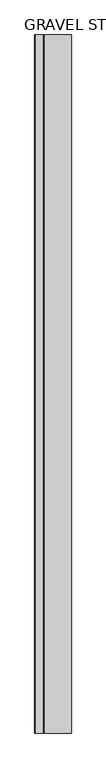
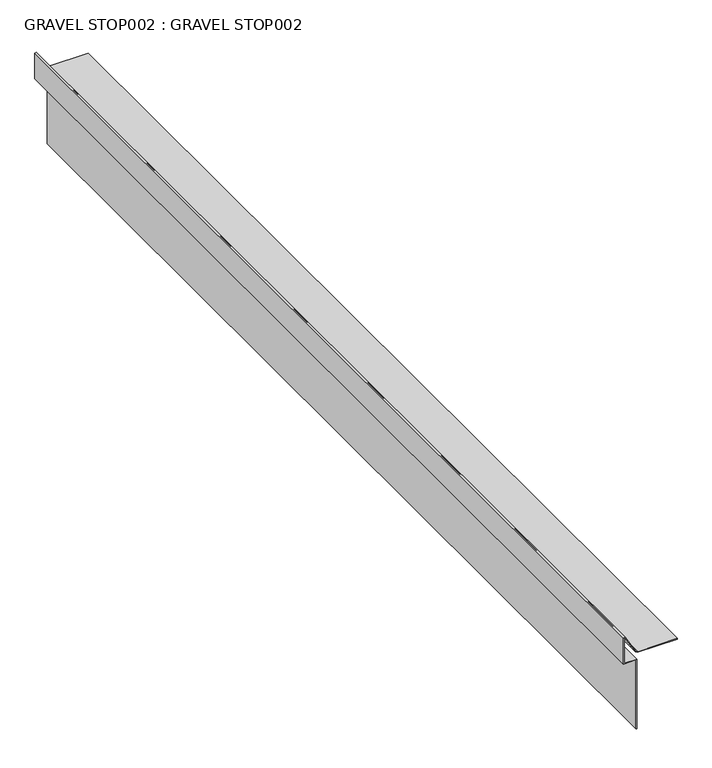
"""IFC4 building model written with IfcOpenShell, lengths in millimetres: proxy geometry, GRAVEL STOP002 : GRAVEL STOP002."""

import ifcopenshell
import ifcopenshell.guid

model = None  # the IFC model being written
_history = None  # IfcOwnerHistory: only IFC2X3 demands one
_inside = {}  # id of a spatial element -> (the spatial element, [elements in it])
_under = {}  # id of a project, library or spatial element -> (it, [spatial elements below it])
_declared = {}  # id of a project -> (the project, [libraries it declares])
_typed = {}  # id of a type object -> (the type object, [elements of that type])
_made_of = {}  # id of a material, layer set ... -> (it, [elements and type objects made of it])


def new_model(schema):
    """Start an empty IFC model of exactly this schema.

    Asked for "IFC4X3", IfcOpenShell would pick the latest addendum, in which some entities
    have other attributes; the version numbers below select the first issue.
    IFC2X3 requires an IfcOwnerHistory on every rooted entity: one is made here for all.
    """
    global model, _history
    if schema == "IFC4X3":
        model = ifcopenshell.file(schema_version=(4, 3, 0, 0))
    else:
        model = ifcopenshell.file(schema=schema)
    _inside.clear()
    _under.clear()
    _declared.clear()
    _typed.clear()
    _made_of.clear()
    _history = None
    if model.schema == "IFC2X3":
        org = make("IfcOrganization", Name="unknown")
        user = make(
            "IfcPersonAndOrganization",
            ThePerson=make("IfcPerson", FamilyName="unknown"),
            TheOrganization=org,
        )
        app = make(
            "IfcApplication",
            ApplicationDeveloper=org,
            Version="unknown",
            ApplicationFullName="unknown",
            ApplicationIdentifier="unknown",
        )
        _history = make(
            "IfcOwnerHistory",
            OwningUser=user,
            OwningApplication=app,
            ChangeAction="ADDED",
            CreationDate=0,
        )
    return model


def make(cls, **values):
    """One entity of the class cls with the attributes given. An attribute that is None is left unset."""
    return model.create_entity(
        cls, **{name: value for name, value in values.items() if value is not None}
    )


def rooted(cls, **values):
    """An entity with a GlobalId (a new one), such as an element, a storey or a relation."""
    return make(cls, GlobalId=ifcopenshell.guid.new(), OwnerHistory=_history, **values)


def si_unit(unit_type, name, prefix=None):
    """IfcSIUnit, for example si_unit("LENGTHUNIT", "METRE", prefix="MILLI")."""
    return make("IfcSIUnit", UnitType=unit_type, Prefix=prefix, Name=name)


def assignment(units):
    """IfcUnitAssignment: the units of a project."""
    return None if units is None else make("IfcUnitAssignment", Units=units)


def point(xyz):
    """IfcCartesianPoint."""
    return None if xyz is None else make("IfcCartesianPoint", Coordinates=xyz)


def direction(xyz):
    """IfcDirection."""
    return None if xyz is None else make("IfcDirection", DirectionRatios=xyz)


def frame(location, z_axis=None, x_axis=None):
    """IfcAxis2Placement3D, a coordinate frame: its origin and axes. An axis left out is left unset."""
    return make(
        "IfcAxis2Placement3D",
        Location=point(location),
        Axis=direction(z_axis),
        RefDirection=direction(x_axis),
    )


def origin():
    """The frame at (0, 0, 0) with its axes left unset."""
    return frame((0.0, 0.0, 0.0))


def place(relative_to, where):
    """IfcLocalPlacement: puts the frame where relative to a parent placement (None: the world)."""
    return make(
        "IfcLocalPlacement", PlacementRelTo=relative_to, RelativePlacement=where
    )


def context(
    kind, dimensions, precision=None, world=None, true_north=None, identifier=None
):
    """IfcGeometricRepresentationContext, for example the 3D "Model" context."""
    return make(
        "IfcGeometricRepresentationContext",
        ContextIdentifier=identifier,
        ContextType=kind,
        CoordinateSpaceDimension=dimensions,
        Precision=precision,
        WorldCoordinateSystem=world,
        TrueNorth=true_north,
    )


def project(units=None, contexts=None):
    """IfcProject with its units and contexts."""
    return rooted(
        "IfcProject",
        Name="project",
        RepresentationContexts=contexts,
        UnitsInContext=assignment(units),
    )


def spatial(cls, under=None, at=None, **own):
    """A site, building, storey or space (cls), placed at a placement, below another one or the project."""
    s = rooted(cls, ObjectPlacement=at, **own)
    if under is not None:
        _under.setdefault(under.id(), (under, []))[1].append(s)
    return s


def polyline(points):
    """IfcPolyline through the points."""
    return make("IfcPolyline", Points=[point(p) for p in points])


def outline(outer, holes=None, kind="AREA"):
    """IfcArbitraryClosedProfileDef: a profile drawn as a closed curve; with holes, ...WithVoids."""
    if holes is None:
        return make("IfcArbitraryClosedProfileDef", ProfileType=kind, OuterCurve=outer)
    return make(
        "IfcArbitraryProfileDefWithVoids",
        ProfileType=kind,
        OuterCurve=outer,
        InnerCurves=holes,
    )


def extrude(swept, where, along, depth):
    """IfcExtrudedAreaSolid: the profile swept, set in the frame where, extruded along a direction by depth."""
    return make(
        "IfcExtrudedAreaSolid",
        SweptArea=swept,
        Position=where,
        ExtrudedDirection=direction(along),
        Depth=depth,
    )


def shape(context_of_items, identifier, shape_type, items):
    """IfcShapeRepresentation: the items that make up one representation, for example the "Body"."""
    return make(
        "IfcShapeRepresentation",
        ContextOfItems=context_of_items,
        RepresentationIdentifier=identifier,
        RepresentationType=shape_type,
        Items=items,
    )


def source(mapping_origin, context_of_items, identifier, shape_type, items):
    """IfcRepresentationMap: a shape defined once, which mapped items show again and again."""
    return make(
        "IfcRepresentationMap",
        MappingOrigin=mapping_origin,
        MappedRepresentation=shape(context_of_items, identifier, shape_type, items),
    )


def transform(
    local_origin,
    x_axis=None,
    y_axis=None,
    z_axis=None,
    scale=None,
    scale2=None,
    scale3=None,
    uniform=True,
):
    """IfcCartesianTransformationOperator3D, or its non-uniform kind. x_axis, y_axis, z_axis: its Axis1, 2, 3."""
    if uniform:
        return make(
            "IfcCartesianTransformationOperator3D",
            Axis1=direction(x_axis),
            Axis2=direction(y_axis),
            LocalOrigin=point(local_origin),
            Scale=scale,
            Axis3=direction(z_axis),
        )
    return make(
        "IfcCartesianTransformationOperator3DnonUniform",
        Axis1=direction(x_axis),
        Axis2=direction(y_axis),
        LocalOrigin=point(local_origin),
        Scale=scale,
        Axis3=direction(z_axis),
        Scale2=scale2,
        Scale3=scale3,
    )


def mapped(mapping_source, mapping_target):
    """IfcMappedItem: shows the shape of a source again, moved by a transform."""
    return make(
        "IfcMappedItem", MappingSource=mapping_source, MappingTarget=mapping_target
    )


def made_of(thing, what):
    """Note that an element or type object is made of a material, layer set ...; save() writes the relation."""
    if what is not None:
        _made_of.setdefault(what.id(), (what, []))[1].append(thing)
    return thing


def element(
    cls,
    number,
    at=None,
    inside=None,
    cuts=None,
    type_object=None,
    material=None,
    context=None,
    identifier="Body",
    shape_type=None,
    held_by="IfcProductDefinitionShape",
    body=None,
    shapes=None,
    **own,
):
    """One element of the class cls, such as IfcWall. Its Tag is "e" and its number.

    at: its placement. inside: the storey or other place that contains it. cuts: it is an
    opening in that element (IfcRelVoidsElement). A single representation is given by context,
    identifier, shape_type and body (its items); several are given by shapes. held_by: the class
    of the entity that holds the representations. save() writes the other relations.
    """
    e = rooted(cls, Tag="e%d" % number, ObjectPlacement=at, **own)
    if body is not None:
        shapes = [shape(context, identifier, shape_type, body)]
    if shapes is not None:
        e.Representation = make(held_by, Representations=shapes)
    if inside is not None:
        _inside.setdefault(inside.id(), (inside, []))[1].append(e)
    if cuts is not None:
        rooted(
            "IfcRelVoidsElement", RelatingBuildingElement=cuts, RelatedOpeningElement=e
        )
    if type_object is not None:
        _typed.setdefault(type_object.id(), (type_object, []))[1].append(e)
    return made_of(e, material)


def aggregate(whole, parts):
    """IfcRelAggregates: a whole, such as a stair, and the parts it consists of."""
    return rooted("IfcRelAggregates", RelatingObject=whole, RelatedObjects=parts)


def save(model, path):
    """Write the relations noted so far, then the file.

    IfcRelAggregates (storeys below a building ...), IfcRelContainedInSpatialStructure (elements
    in a storey), IfcRelDefinesByType, IfcRelAssociatesMaterial and IfcRelDeclares: one each for
    every whole, place, type object, material and project.
    """
    for whole, parts in _under.values():
        aggregate(whole, parts)
    for where, things in _inside.values():
        rooted(
            "IfcRelContainedInSpatialStructure",
            RelatedElements=things,
            RelatingStructure=where,
        )
    for kind, things in _typed.values():
        rooted("IfcRelDefinesByType", RelatedObjects=things, RelatingType=kind)
    for what, things in _made_of.values():
        rooted("IfcRelAssociatesMaterial", RelatedObjects=things, RelatingMaterial=what)
    for by, libraries in _declared.values():
        rooted("IfcRelDeclares", RelatingContext=by, RelatedDefinitions=libraries)
    model.write(path)


def gravel_stop002_gravel_stop002_21b18a30(model_context):
    return source(origin(), model_context, "Body", "SweptSolid", [
        extrude(outline(polyline([(40295.3431515, -5034.9087762), (40294.5307525, -5037.9406906), (40240.9633674, -5037.9406906), (40240.9633674, -5013.600953), (40097.9858473, -5013.600953), (40097.9858473, -5012.189842), (40242.3744784, -5012.189842), (40242.3744784, -5036.5295796), (40293.447969, -5036.5295796), (40293.699878, -5035.5894424), (40258.5078708, -5015.2713276), (40255.9633674, -5010.8641185), (40255.9633674, -4933.0281058), (40257.3744784, -4933.0281058), (40257.3744784, -5010.4860124), (40259.5408757, -5014.2383227), (40295.3431515, -5034.9087762)])), frame((0.0, -1052.8906573, 0.0), z_axis=(0.0, 1.0, 0.0), x_axis=(0.0, 0.0, 1.0)), (0.0, 0.0, 1.0), 2000.25),
    ])


if __name__ == "__main__":
    model = new_model("IFC4")
    model_context = context("Model", 3, world=origin())
    ifc_project = project(units=[si_unit("LENGTHUNIT", "METRE", prefix="MILLI")], contexts=[model_context])
    site = spatial("IfcSite", under=ifc_project)
    building = spatial("IfcBuilding", under=site)
    placement = place(None, origin())
    gravel_stop002_gravel_stop002_shape = gravel_stop002_gravel_stop002_21b18a30(model_context)
    element("IfcBuildingElementProxy", 1, Name="GRAVEL STOP002 : GRAVEL STOP002", ObjectType="GRAVEL STOP002 : GRAVEL STOP002", at=placement, inside=building, context=model_context, shape_type="MappedRepresentation", body=[
        mapped(gravel_stop002_gravel_stop002_shape, transform((0.0, 0.0, 0.0), x_axis=(1.0, 0.0, 0.0), y_axis=(0.0, 1.0, 0.0), z_axis=(0.0, 0.0, 1.0))),
    ])
    save(model, "model.ifc")

# Revit data of these elements
# Type "GRAVEL STOP002 : GRAVEL STOP002"
#   NameOverride = "GRAVEL STOP002"
# Element 1 (IfcBuildingElementProxy, "GRAVEL STOP002 : GRAVEL STOP002")
#   Materials on its faces: "GRAVEL STOP REQUIRED WITH GRAVEL SURFACE SYSTEMS"
# Materials
#   "GRAVEL STOP REQUIRED WITH GRAVEL SURFACE SYSTEMS": class "Unassigned", colour RGB 170 170 127, transparency 0, Cost = 0
